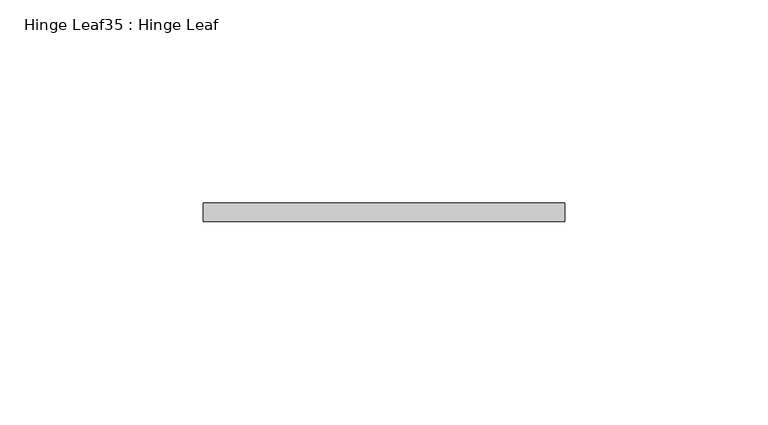
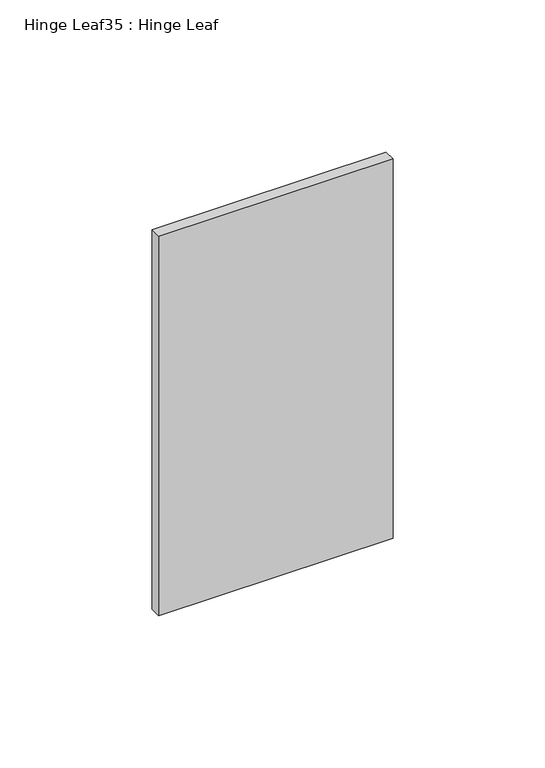
"""IFC4 building model written with IfcOpenShell, lengths in millimetres: proxy geometry, Hinge Leaf35 : Hinge Leaf."""

from ifc_helpers import new_model, si_unit, frame, origin, place, context, project, spatial, polyline, outline, extrude, source, transform, mapped, element, save


def hinge_leaf35_hinge_leaf_49d9ed16(model_context):
    return source(origin(), model_context, "Body", "SweptSolid", [
        extrude(outline(polyline([(587327.7934739, -533988.7163841), (587327.7934739, -533984.1443841), (587416.6934739, -533984.1443841), (587416.6934739, -533988.7163841), (587327.7934739, -533988.7163841)])), frame((0.0, 0.0, 1936.75), z_axis=(0.0, 0.0, 1.0), x_axis=(1.0, 0.0, 0.0)), (0.0, 0.0, 1.0), 152.4),
    ])


if __name__ == "__main__":
    model = new_model("IFC4")
    model_context = context("Model", 3, world=origin())
    ifc_project = project(units=[si_unit("LENGTHUNIT", "METRE", prefix="MILLI")], contexts=[model_context])
    site = spatial("IfcSite", under=ifc_project)
    building = spatial("IfcBuilding", under=site)
    placement = place(None, origin())
    hinge_leaf35_hinge_leaf_shape = hinge_leaf35_hinge_leaf_49d9ed16(model_context)
    element("IfcBuildingElementProxy", 1, Name="Hinge Leaf35 : Hinge Leaf", ObjectType="Hinge Leaf35 : Hinge Leaf", at=placement, inside=building, context=model_context, shape_type="MappedRepresentation", body=[
        mapped(hinge_leaf35_hinge_leaf_shape, transform((0.0, 0.0, 0.0), x_axis=(1.0, 0.0, 0.0), y_axis=(0.0, 1.0, 0.0), z_axis=(0.0, 0.0, 1.0))),
    ])
    save(model, "model.ifc")

# Revit data of these elements
# Element 1 (IfcBuildingElementProxy, "Hinge Leaf35 : Hinge Leaf")
#   Materials on its faces: "6\"X6\" WELD-ON STL BUTT HINGE"
# Materials
#   "6\"X6\" WELD-ON STL BUTT HINGE": class "Metal", colour RGB 189 187 185, transparency 0, Description = "Carbon steel", Cost = 0
